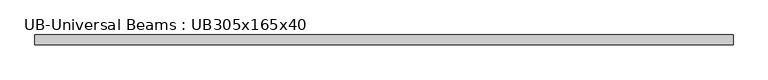
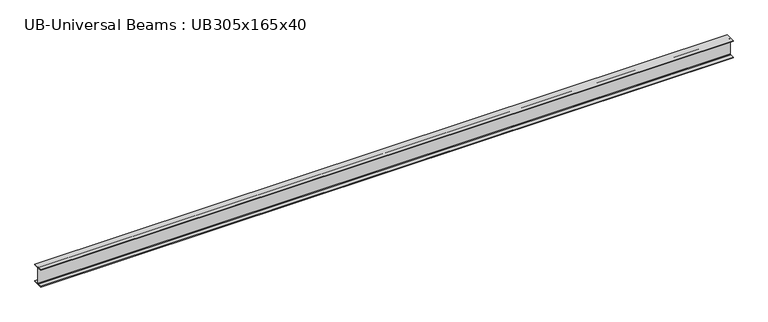
"""IFC4 building model written with IfcOpenShell, lengths in millimetres: member geometry, UB-Universal Beams : UB305x165x40."""

from ifc_helpers import new_model, si_unit, point, frame, frame_2d, origin, place, context, project, spatial, polyline, circle_curve, trimmed, segment, composite_curve, outline, extrude, source, transform, mapped, element, save


def ub_universal_beams_ub305x165x40_035d116d(model_context):
    return source(origin(), model_context, "Body", "SweptSolid", [
        extrude(outline(composite_curve([segment(polyline([(82.5, -141.5), (82.5, -151.7), (-82.5, -151.7), (-82.5, -141.5), (-11.9, -141.5)]), True, "CONTINUOUS"), segment(trimmed(circle_curve(frame_2d((-11.9, -132.6)), 8.9), [point((-11.9, -141.5))], [point((-3.0, -132.6))], True, "CARTESIAN"), True, "CONTINUOUS"), segment(polyline([(-3.0, -132.6), (-3.0, 132.6)]), True, "CONTINUOUS"), segment(trimmed(circle_curve(frame_2d((-11.9, 132.6)), 8.9), [point((-3.0, 132.6))], [point((-11.9, 141.5))], True, "CARTESIAN"), True, "CONTINUOUS"), segment(polyline([(-11.9, 141.5), (-82.5, 141.5), (-82.5, 151.7), (82.5, 151.7), (82.5, 141.5), (11.9, 141.5)]), True, "CONTINUOUS"), segment(trimmed(circle_curve(frame_2d((11.9, 132.6)), 8.9), [point((11.9, 141.5))], [point((3.0, 132.6))], True, "CARTESIAN"), True, "CONTINUOUS"), segment(polyline([(3.0, 132.6), (3.0, -132.6)]), True, "CONTINUOUS"), segment(trimmed(circle_curve(frame_2d((11.9, -132.6)), 8.9), [point((3.0, -132.6))], [point((11.9, -141.5))], True, "CARTESIAN"), True, "CONTINUOUS"), segment(polyline([(11.9, -141.5), (82.5, -141.5)]), True, "CONTINUOUS")], self_intersect=False)), frame((-5621.65, 0.0, 0.0), z_axis=(1.0, 0.0, 0.0), x_axis=(0.0, 1.0, 0.0)), (0.0, 0.0, 1.0), 11577.5),
    ])


if __name__ == "__main__":
    model = new_model("IFC4")
    model_context = context("Model", 3, world=origin())
    ifc_project = project(units=[si_unit("LENGTHUNIT", "METRE", prefix="MILLI")], contexts=[model_context])
    site = spatial("IfcSite", under=ifc_project)
    building = spatial("IfcBuilding", under=site)
    placement = place(None, origin())
    ub_universal_beams_ub305x165x40_shape = ub_universal_beams_ub305x165x40_035d116d(model_context)
    element("IfcMember", 1, ObjectType="UB-Universal Beams : UB305x165x40", at=placement, inside=building, context=model_context, shape_type="MappedRepresentation", body=[
        mapped(ub_universal_beams_ub305x165x40_shape, transform((0.0, 0.0, 0.0), x_axis=(1.0, 0.0, 0.0), y_axis=(0.0, 1.0, 0.0), z_axis=(0.0, 0.0, 1.0))),
    ])
    save(model, "model.ifc")

# Revit data of these elements
# Type "UB-Universal Beams : UB305x165x40"
#   Section Name Key = "UB305X165X40"
#   Width = 16.5 cm
#   Web Thickness = 0.6 cm
#   Web Fillet = 0.89 cm
#   Warping Constant = 164000.0 cm⁶
#   Torsional Moment of Inertia = 14.70 cm⁴
#   Section Area = 51.3 cm²
#   Plastic Modulus weak axis = 142.0 cm³
#   Plastic Modulus strong axis = 623.0 cm³
#   Nominal Weight = 40.2999 kgf/m
#   Moment of Inertia weak axis = 764.00 cm⁴
#   Moment of Inertia strong axis = 8503.00 cm⁴
#   Height = 30.34 cm
#   Flange Thickness = 1.02 cm
#   Elastic Modulus weak axis = 92.6 cm³
#   Elastic Modulus strong axis = 560.0 cm³
#   Centroid Vertical = 15.17 cm
#   Centroid Horizontal = 8.25 cm
#   Bolt Spacing = 9.0 cm
#   Length [instance default] = 1500 mm
#   Structural Material [instance default] = Metal - Steel 43-275
#   Type Comments = ""
#   Assembly Code = ""
# Element 1 (IfcMember, "UB-Universal Beams : UB305x165x40")
#   Materials on its faces: "Metal - Steel 43-275"
# Materials
#   "Metal - Steel 43-275": class "Metal", colour RGB 247 247 247, transparency 0, Cost = 0
